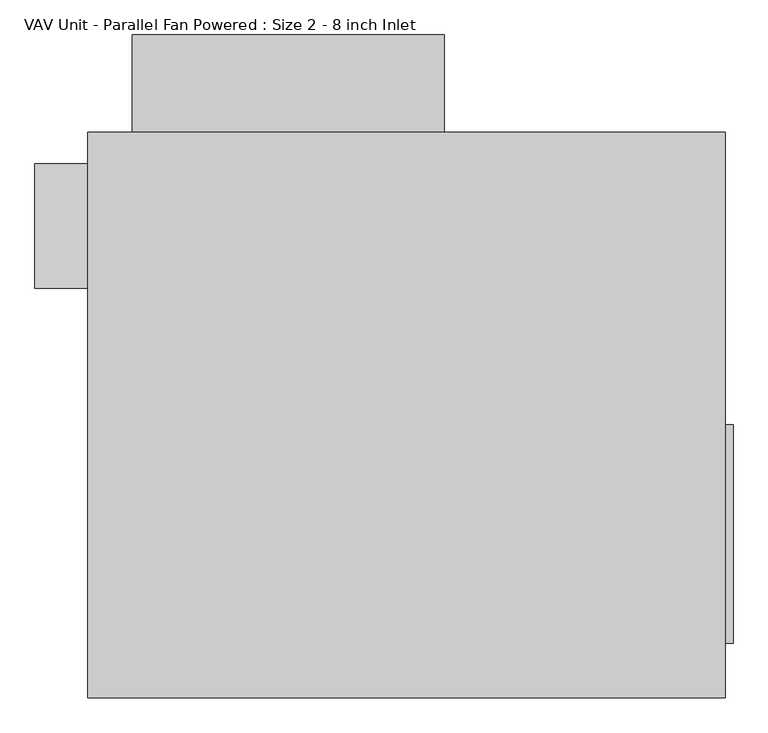
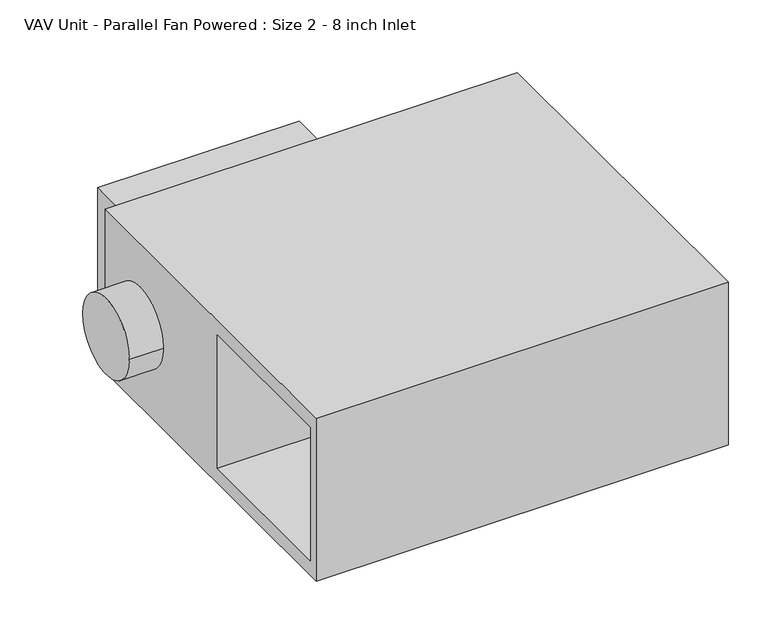
"""IFC4 building model written with IfcOpenShell, lengths in millimetres: proxy geometry, VAV Unit - Parallel Fan Powered : Size 2 - 8 inch Inlet."""

from ifc_helpers import new_model, si_unit, point, frame, frame_2d, origin, place, context, project, spatial, polyline, circle_curve, trimmed, segment, composite_curve, outline, extrude, faceted_brep, source, transform, mapped, element, save


def vav_unit_parallel_fan_powered_size_2_8_inch_inlet_1779b90c(model_context):
    return source(origin(), model_context, "Body", "SolidModel", [
        extrude(outline(polyline([(531.8125, -15.875), (531.8125, -371.475), (519.1125, -371.475), (519.1125, -15.875), (531.8125, -15.875)])), frame((0.0, 0.0, -139.7), z_axis=(0.0, 0.0, 1.0), x_axis=(1.0, 0.0, 0.0)), (0.0, 0.0, 1.0), 279.4),
        extrude(outline(polyline([(61.9125, 460.375), (-446.0875, 460.375), (-446.0875, 619.125), (61.9125, 619.125), (61.9125, 460.375)])), frame((0.0, 0.0, -152.4), z_axis=(0.0, 0.0, 1.0), x_axis=(1.0, 0.0, 0.0)), (0.0, 0.0, 1.0), 304.8),
        extrude(outline(composite_curve([segment(trimmed(circle_curve(frame_2d((307.975, 0.0)), 101.6), [point((206.375, 0.0))], [point((409.575, 0.0))], False, "CARTESIAN"), True, "CONTINUOUS"), segment(trimmed(circle_curve(frame_2d((307.975, 0.0)), 101.6), [point((409.575, 0.0))], [point((206.375, 0.0))], False, "CARTESIAN"), True, "CONTINUOUS")], self_intersect=False)), frame((-604.8375, 0.0, 0.0), z_axis=(1.0, 0.0, 0.0), x_axis=(0.0, 1.0, 0.0)), (0.0, 0.0, 1.0), 85.725),
        faceted_brep([(519.1125, 460.375, 217.4875), (-519.1125, 460.375, 217.4875), (-519.1125, -460.375, 217.4875), (519.1125, -460.375, 217.4875), (519.1125, 460.375, -217.4875), (519.1125, -460.375, -217.4875), (-519.1125, -460.375, -217.4875), (-519.1125, 460.375, -217.4875), (-519.1125, -434.975, 177.8), (-519.1125, -434.975, -177.8), (-519.1125, -28.575, -177.8), (-519.1125, -28.575, 177.8), (0.0, -434.975, 177.8), (0.0, -28.575, 177.8), (0.0, -28.575, -177.8), (0.0, -434.975, -177.8)], [[[0, 1, 2, 3]], [[4, 5, 6, 7]], [[1, 0, 4, 7]], [[2, 1, 7, 6], [8, 9, 10, 11]], [[3, 2, 6, 5]], [[0, 3, 5, 4]], [[12, 13, 14, 15]], [[12, 15, 9, 8]], [[15, 14, 10, 9]], [[14, 13, 11, 10]], [[13, 12, 8, 11]]]),
    ])


if __name__ == "__main__":
    model = new_model("IFC4")
    model_context = context("Model", 3, world=origin())
    ifc_project = project(units=[si_unit("LENGTHUNIT", "METRE", prefix="MILLI")], contexts=[model_context])
    site = spatial("IfcSite", under=ifc_project)
    building = spatial("IfcBuilding", under=site)
    placement = place(None, origin())
    vav_unit_parallel_fan_powered_size_2_8_inch_inlet_shape = vav_unit_parallel_fan_powered_size_2_8_inch_inlet_1779b90c(model_context)
    element("IfcBuildingElementProxy", 1, Name="VAV Unit - Parallel Fan Powered : Size 2 - 8 inch Inlet", ObjectType="VAV Unit - Parallel Fan Powered : Size 2 - 8 inch Inlet", at=placement, inside=building, context=model_context, shape_type="MappedRepresentation", body=[
        mapped(vav_unit_parallel_fan_powered_size_2_8_inch_inlet_shape, transform((0.0, 0.0, 0.0), x_axis=(1.0, 0.0, 0.0), y_axis=(0.0, 1.0, 0.0), z_axis=(0.0, 0.0, 1.0))),
    ])
    save(model, "model.ifc")

# Revit data of these elements
# Type "VAV Unit - Parallel Fan Powered : Size 2 - 8 inch Inlet"
#   Width2 = 1' - 2"
#   Voltage = 120 V
#   UnitWidth = 3' - 4 7/8"
#   UnitHeight = 3' - 0 1/4"
#   UnitDepth = 1' - 5 1/8"
#   SupplyConnectorWidth = 1' - 2"
#   SupplyConnectorVerticalOffset = 0' - 2 1/8"
#   SupplyConnectorLength = 0' - 0 1/2"
#   SupplyConnectorHorizontalOffset = 0' - 3 1/2"
#   SupplyConnectorDepth = 0' - 11"
#   SupplyAirConnectorCenterOffset = 0' - 10 1/2"
#   PrimaryToSupplyRatio [instance default] = 0.2
#   PrimaryAirOffset = 0' - 6"
#   PrimaryAirFlow [instance default] = 180 CFM
#   PrimaryAirConnectorVerticalOffset = 0' - 8 9/16"
#   PrimaryAirConnectorRadius = 0' - 4"
#   PrimaryAirConnectorLength = 0' - 3 3/8"
#   PrimaryAirConnectorDiameter = 0' - 8"
#   PrimaryAirConnectorCenterOffset = 0' - 6"
#   Pressure Drop [instance default] = 0.02 in-wg
#   InducedAirInletWidth = 1' - 4"
#   InducedAirInletDepth = 1' - 2"
#   InducedAirConnectorHorizontalOffset = 0' - 1"
#   InducedAirConnectorCenterOffset = 0' - 9"
#   Height2 = 0' - 11"
#   ElectricalConnectionBoxWidth = 1' - 8"
#   ElectricalConnectionBoxOffset = 0' - 2 7/8"
#   ElectricalConnectionBoxHeight = 0' - 6 1/4"
#   ElectricalConnectionBoxDepth = 1' - 0"
#   SupplyAirFlow [instance default] = 900 CFM
#   Apparent Load = 271 VA
#   SupplyAirConnectorIndex = 2
#   PrimaryAirConnectorIndex = 1
#   Number of Poles = 1
#   InducedAirConnectorIndex = 3
#   VAV Material = none
#   Load Classification = Cooling
#   Default Elevation = 0
#   Assembly Code = ""
